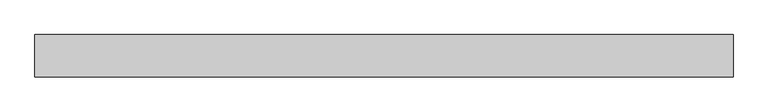
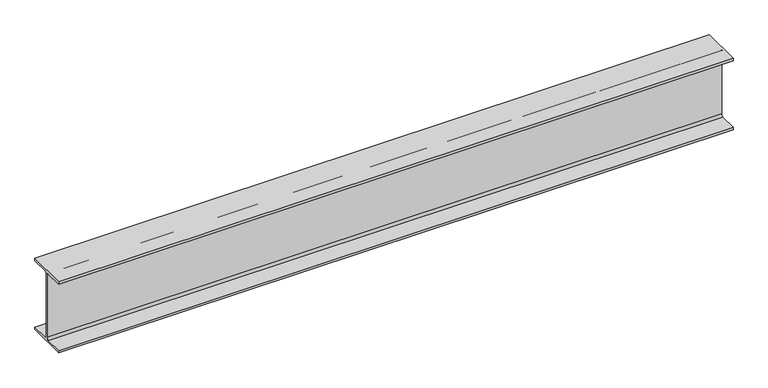
"""IFC4 building model written with IfcOpenShell, lengths in millimetres: beam geometry, Old_Steel Beam_H-KSD3502 : H_SB_ASB_H-194×150x6x9."""

from ifc_helpers import new_model, si_unit, point, frame, frame_2d, origin, place, context, project, spatial, polyline, circle_curve, trimmed, segment, composite_curve, outline, extrude, source, transform, mapped, element, save


def beam_e3063bc9(model_context):
    return source(origin(), model_context, "Body", "SweptSolid", [
        extrude(outline(composite_curve([segment(polyline([(-82.5, -141.5), (-11.9, -141.5)]), True, "CONTINUOUS"), segment(trimmed(circle_curve(frame_2d((-11.9, -132.6)), 8.9), [point((-11.9, -141.5))], [point((-3.0, -132.6))], True, "CARTESIAN"), True, "CONTINUOUS"), segment(polyline([(-3.0, -132.6), (-3.0, 132.6)]), True, "CONTINUOUS"), segment(trimmed(circle_curve(frame_2d((-11.9, 132.6)), 8.9), [point((-3.0, 132.6))], [point((-11.9, 141.5))], True, "CARTESIAN"), True, "CONTINUOUS"), segment(polyline([(-11.9, 141.5), (-82.5, 141.5), (-82.5, 151.7), (82.5, 151.7), (82.5, 141.5), (11.9, 141.5)]), True, "CONTINUOUS"), segment(trimmed(circle_curve(frame_2d((11.9, 132.6)), 8.9), [point((11.9, 141.5))], [point((3.0, 132.6))], True, "CARTESIAN"), True, "CONTINUOUS"), segment(polyline([(3.0, 132.6), (3.0, -132.6)]), True, "CONTINUOUS"), segment(trimmed(circle_curve(frame_2d((11.9, -132.6)), 8.9), [point((3.0, -132.6))], [point((11.9, -141.5))], True, "CARTESIAN"), True, "CONTINUOUS"), segment(polyline([(11.9, -141.5), (82.5, -141.5), (82.5, -151.7), (-82.5, -151.7), (-82.5, -141.5)]), True, "CONTINUOUS")], self_intersect=False)), frame((-1579.8617116, 0.0, 0.0), z_axis=(1.0, 0.0, 0.0), x_axis=(0.0, 1.0, 0.0)), (0.0, 0.0, 1.0), 2719.057388),
    ])


if __name__ == "__main__":
    model = new_model("IFC4")
    model_context = context("Model", 3, world=origin())
    ifc_project = project(units=[si_unit("LENGTHUNIT", "METRE", prefix="MILLI")], contexts=[model_context])
    site = spatial("IfcSite", under=ifc_project)
    building = spatial("IfcBuilding", under=site)
    placement = place(None, origin())
    beam_shape = beam_e3063bc9(model_context)
    element("IfcBeam", 1, ObjectType="Old_Steel Beam_H-KSD3502 : H_SB_ASB_H-194×150x6x9", at=placement, inside=building, context=model_context, shape_type="MappedRepresentation", body=[
        mapped(beam_shape, transform((0.0, 0.0, 0.0), x_axis=(1.0, 0.0, 0.0), y_axis=(0.0, 1.0, 0.0), z_axis=(0.0, 0.0, 1.0))),
    ])
    save(model, "model.ifc")

# Revit data of these elements
# Type "Old_Steel Beam_H-KSD3502 : H_SB_ASB_H-194×150x6x9"
#   Width = 15.0 cm
#   Web Thickness = 0.6 cm
#   Web Fillet = 1.3 cm
#   Warping Constant = 43316.0 cm⁶
#   Torsional Moment of Inertia = 8.622 cm⁴
#   Torsional Modulus = 1.0 cm³
#   Section Area = 39.01 cm²
#   Plastic Modulus weak axis = 104.0 cm³
#   Plastic Modulus strong axis = 309.0 cm³
#   Perimeter = 0.95 m²/m
#   Nominal Weight = 30.60 kgf/m
#   Moment of Inertia weak axis = 507.00 cm⁴
#   Moment of Inertia strong axis = 2690.00 cm⁴
#   Height = 19.4 cm
#   Flange Thickness = 0.9 cm
#   Elastic Modulus weak axis = 67.6 cm³
#   Elastic Modulus strong axis = 277.0 cm³
#   Centroid Vertical = 9.7 cm
#   Centroid Horizontal = 7.5 cm
#   Length [instance default] = 1.5240 m
#   Structural Material [instance default] = Steel, 45-345
#   Assembly Code = ""
# Element 1 (IfcBeam, "Old_Steel Beam_H-KSD3502 : H_SB_ASB_H-194×150x6x9")
#   Structural Material = none
# Materials
#   "Steel, 45-345": class "Metal", colour RGB 189 187 185, transparency 0, Description = "Steel 345 MPa", Cost = 0
